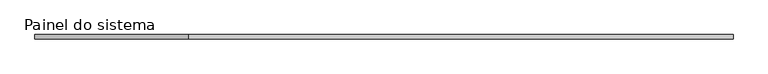
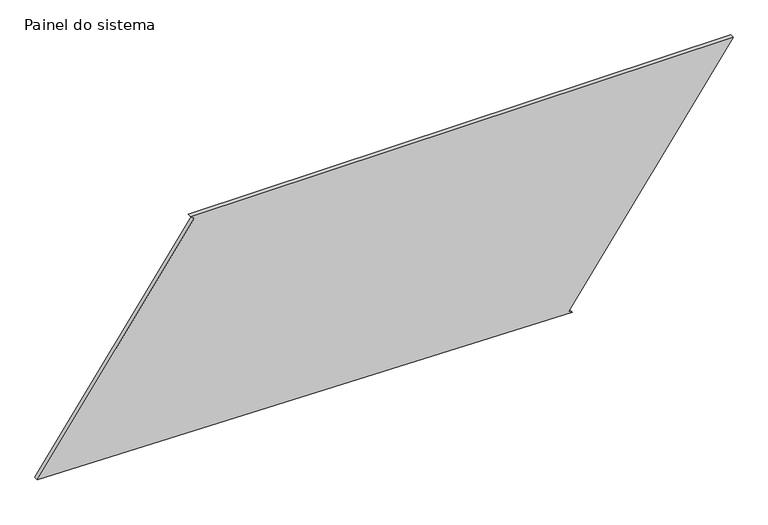
"""IFC4 building model written with IfcOpenShell, lengths in millimetres: plate geometry, Painel do sistema : Envidraçado."""

from ifc_helpers import new_model, si_unit, frame, origin, place, context, project, spatial, polyline, outline, extrude, source, transform, mapped, element, save


def painel_do_sistema_53fe73f6(model_context):
    return source(origin(), model_context, "Body", "SweptSolid", [
        extrude(outline(polyline([(0.0, 1076.7945905), (14.4529738, 1056.3957781), (1350.3753306, 2002.9239601), (1350.3753306, -1119.3520894), (1335.9223568, -1098.953277), (60.0653158, -2002.9239601), (0.0, 1076.7945905)])), frame((0.0, 24.5, 0.0), z_axis=(0.0, 1.0, 0.0), x_axis=(0.0, 0.0, 1.0)), (0.0, 0.0, 1.0), 25.0),
    ])


if __name__ == "__main__":
    model = new_model("IFC4")
    model_context = context("Model", 3, world=origin())
    ifc_project = project(units=[si_unit("LENGTHUNIT", "METRE", prefix="MILLI")], contexts=[model_context])
    site = spatial("IfcSite", under=ifc_project)
    building = spatial("IfcBuilding", under=site)
    placement = place(None, origin())
    painel_do_sistema_shape = painel_do_sistema_53fe73f6(model_context)
    element("IfcPlate", 1, ObjectType="Painel do sistema : Envidraçado", at=placement, inside=building, context=model_context, shape_type="MappedRepresentation", body=[
        mapped(painel_do_sistema_shape, transform((0.0, 0.0, 0.0), x_axis=(1.0, 0.0, 0.0), y_axis=(0.0, 1.0, 0.0), z_axis=(0.0, 0.0, 1.0))),
    ])
    save(model, "model.ifc")

# Revit data of these elements
# Type "Painel do sistema : Envidraçado"
#   Construction Type Id = "GSP4R"
#   Analytic Construction = "Vidraça única Pilkington 1/8 pol"
#   Visual Light Transmittance = 0.9
#   Solar Heat Gain Coefficient = 0.86
#   Heat Transfer Coefficient (U) = 6.7069 W/(m²·K)
# Element 1 (IfcPlate, "Painel do sistema : Envidraçado")
#   Materials on its faces: "Vidro"
# Materials
#   "Vidro": class "Vidro", colour RGB 0 128 192, transparency 0.9, Description = "Vidro de sílica", Cost = 0
